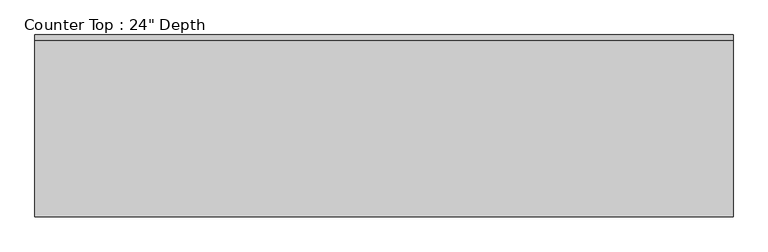
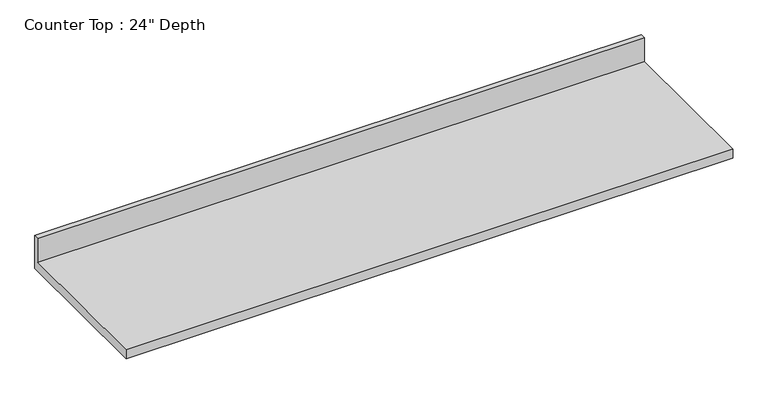
"""IFC4 building model written with IfcOpenShell, lengths in millimetres: furniture geometry."""

from ifc_helpers import new_model, si_unit, frame, origin, place, context, project, spatial, polyline, outline, extrude, source, transform, mapped, element, save


def furniture_deb1c5d1(model_context):
    return source(origin(), model_context, "Body", "SweptSolid", [
        extrude(outline(polyline([(0.0, 1016.0), (0.0, 876.3), (-635.0, 876.3), (-635.0, 914.4), (-19.05, 914.4), (-19.05, 1016.0), (0.0, 1016.0)])), frame((-1200.4622951, 0.0, 0.0), z_axis=(1.0, 0.0, 0.0), x_axis=(0.0, 1.0, 0.0)), (0.0, 0.0, 1.0), 2438.4),
    ])


if __name__ == "__main__":
    model = new_model("IFC4")
    model_context = context("Model", 3, world=origin())
    ifc_project = project(units=[si_unit("LENGTHUNIT", "METRE", prefix="MILLI")], contexts=[model_context])
    site = spatial("IfcSite", under=ifc_project)
    building = spatial("IfcBuilding", under=site)
    placement = place(None, origin())
    furniture_shape = furniture_deb1c5d1(model_context)
    element("IfcFurniture", 1, ObjectType="Counter Top : 24\" Depth", at=placement, inside=building, context=model_context, shape_type="MappedRepresentation", body=[
        mapped(furniture_shape, transform((0.0, 0.0, 0.0), x_axis=(1.0, 0.0, 0.0), y_axis=(0.0, 1.0, 0.0), z_axis=(0.0, 0.0, 1.0))),
    ])
    save(model, "model.ifc")

# Revit data of these elements
# Type "Counter Top : 24\" Depth"
#   Assembly Code = "C1030400"
#   Counter Thickness = 0' - 1 1/2"
#   Depth = 2' - 1"
#   Height = 3' - 0"
#   Length [instance default] = 8' - 0"
#   Counter Top Material = none
#   Default Elevation = 0
# Element 1 (IfcFurniture, "Counter Top : 24\" Depth")
#   Materials on its faces: "Laminate"
# Materials
#   "Laminate": class "Unassigned", colour RGB 247 235 201, transparency 0
